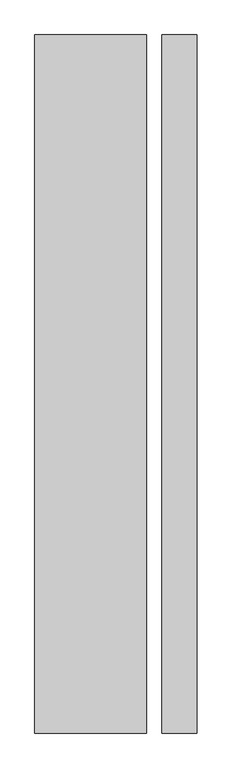
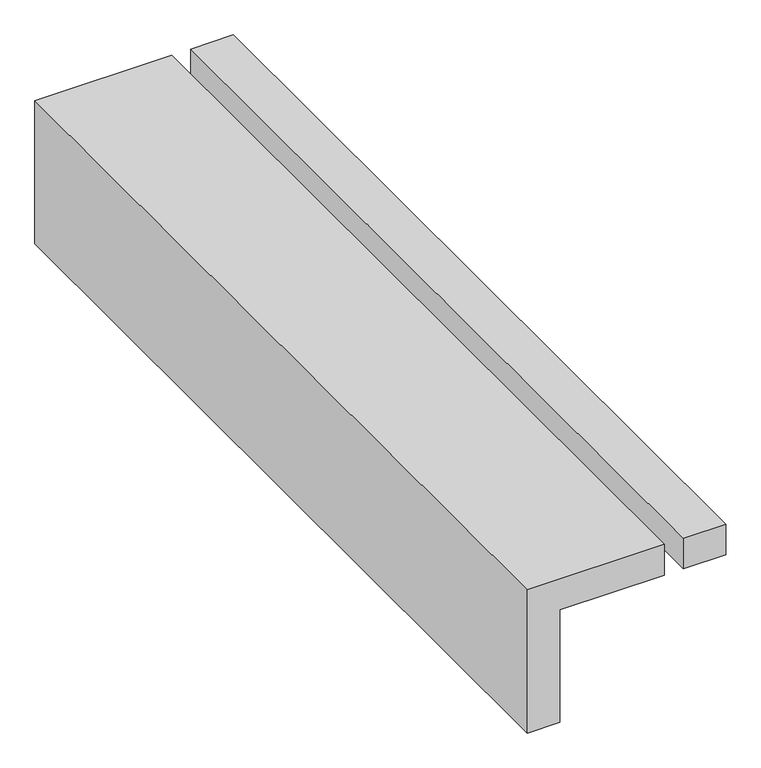
"""IFC4 building model written with IfcOpenShell, lengths in millimetres: proxy geometry, Framing062 4:Framing062 15035:304927 : Framing062 4:Framing062 15035:304927."""

from ifc_helpers import new_model, si_unit, frame, origin, place, context, project, spatial, polyline, outline, extrude, source, transform, mapped, element, save


def generic_models_af73d8aa(model_context):
    return source(origin(), model_context, "Body", "SweptSolid", [
        extrude(outline(polyline([(4302.7564157, 1225.4418837), (4302.7564157, -774.5581163), (4202.8571994, -774.5581163), (4202.8571994, 1225.4418837), (4302.7564157, 1225.4418837)])), frame((0.0, 0.0, 42413.2036692), z_axis=(0.0, 0.0, 1.0), x_axis=(1.0, 0.0, 0.0)), (0.0, 0.0, 1.0), 76.2),
        extrude(outline(polyline([(42134.105552, 3837.4205383), (42134.105552, 3913.6205383), (42413.2036692, 3913.6205383), (42413.2036692, 4158.4071994), (42489.4036692, 4158.4071994), (42489.4036692, 3837.4205383), (42134.105552, 3837.4205383)])), frame((0.0, -774.5581163, 0.0), z_axis=(0.0, 1.0, 0.0), x_axis=(0.0, 0.0, 1.0)), (0.0, 0.0, 1.0), 2000.0),
    ])


if __name__ == "__main__":
    model = new_model("IFC4")
    model_context = context("Model", 3, world=origin())
    ifc_project = project(units=[si_unit("LENGTHUNIT", "METRE", prefix="MILLI")], contexts=[model_context])
    site = spatial("IfcSite", under=ifc_project)
    building = spatial("IfcBuilding", under=site)
    placement = place(None, origin())
    generic_models_shape = generic_models_af73d8aa(model_context)
    element("IfcBuildingElementProxy", 1, Name="Framing062 4:Framing062 15035:304927 : Framing062 4:Framing062 15035:304927", ObjectType="Framing062 4:Framing062 15035:304927 : Framing062 4:Framing062 15035:304927", at=placement, inside=building, context=model_context, shape_type="MappedRepresentation", body=[
        mapped(generic_models_shape, transform((0.0, 0.0, 0.0), x_axis=(1.0, 0.0, 0.0), y_axis=(0.0, 1.0, 0.0), z_axis=(0.0, 0.0, 1.0))),
    ])
    save(model, "model.ifc")

# Revit data of these elements
# Type "Framing062 4:Framing062 15035:304927 : Framing062 4:Framing062 15035:304927"
#   NameOverride = "Framing062 4:Framing062 15035:304927"
#   ObjectTypeOverride = "Framing062 4:Framing062 15035"
#   Reference = "Framing062 15035"
#   Category = "Generic Models"
#   Tag = "304927"
# Element 1 (IfcBuildingElementProxy, "Framing062 4:Framing062 15035:304927 : Framing062 4:Framing062 15035:304927")
#   Materials on its faces: "POLYURETHANE SPRAY FOAM UNDER ROOF SUBSTRATE (SEE T-24 ENERGY REPORT FOR R-VALUE)"
# Materials
#   "POLYURETHANE SPRAY FOAM UNDER ROOF SUBSTRATE (SEE T-24 ENERGY REPORT FOR R-VALUE)": class "Unassigned", colour RGB 210 164 194, transparency 0, Cost = 0
